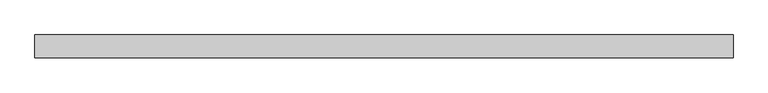
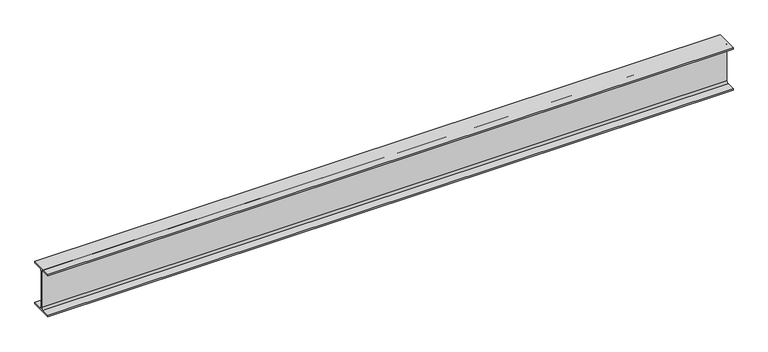
"""IFC4 building model written with IfcOpenShell, lengths in millimetres: beam geometry, 0912_Steel Framing_H-KSD3502 : H_SB_ASB_H-250x125x6x9."""

from ifc_helpers import new_model, si_unit, point, frame, frame_2d, origin, place, context, project, spatial, polyline, circle_curve, trimmed, segment, composite_curve, outline, extrude, source, transform, mapped, element, save


def beam_51e572f2(model_context):
    return source(origin(), model_context, "Body", "SweptSolid", [
        extrude(outline(composite_curve([segment(polyline([(62.5, -116.0), (62.5, -125.0), (-62.5, -125.0), (-62.5, -116.0), (-15.0, -116.0)]), True, "CONTINUOUS"), segment(trimmed(circle_curve(frame_2d((-15.0, -104.0)), 12.0), [point((-15.0, -116.0))], [point((-3.0, -104.0))], True, "CARTESIAN"), True, "CONTINUOUS"), segment(polyline([(-3.0, -104.0), (-3.0, 104.0)]), True, "CONTINUOUS"), segment(trimmed(circle_curve(frame_2d((-15.0, 104.0)), 12.0), [point((-3.0, 104.0))], [point((-15.0, 116.0))], True, "CARTESIAN"), True, "CONTINUOUS"), segment(polyline([(-15.0, 116.0), (-62.5, 116.0), (-62.5, 125.0), (62.5, 125.0), (62.5, 116.0), (15.0, 116.0)]), True, "CONTINUOUS"), segment(trimmed(circle_curve(frame_2d((15.0, 104.0)), 12.0), [point((15.0, 116.0))], [point((3.0, 104.0))], True, "CARTESIAN"), True, "CONTINUOUS"), segment(polyline([(3.0, 104.0), (3.0, -104.0)]), True, "CONTINUOUS"), segment(trimmed(circle_curve(frame_2d((15.0, -104.0)), 12.0), [point((3.0, -104.0))], [point((15.0, -116.0))], True, "CARTESIAN"), True, "CONTINUOUS"), segment(polyline([(15.0, -116.0), (62.5, -116.0)]), True, "CONTINUOUS")], self_intersect=False)), frame((-1904.8, 0.0, 0.0), z_axis=(1.0, 0.0, 0.0), x_axis=(0.0, 1.0, 0.0)), (0.0, 0.0, 1.0), 3809.6),
    ])


if __name__ == "__main__":
    model = new_model("IFC4")
    model_context = context("Model", 3, world=origin())
    ifc_project = project(units=[si_unit("LENGTHUNIT", "METRE", prefix="MILLI")], contexts=[model_context])
    site = spatial("IfcSite", under=ifc_project)
    building = spatial("IfcBuilding", under=site)
    placement = place(None, origin())
    beam_shape = beam_51e572f2(model_context)
    element("IfcBeam", 1, ObjectType="0912_Steel Framing_H-KSD3502 : H_SB_ASB_H-250x125x6x9", at=placement, inside=building, context=model_context, shape_type="MappedRepresentation", body=[
        mapped(beam_shape, transform((0.0, 0.0, 0.0), x_axis=(1.0, 0.0, 0.0), y_axis=(0.0, 1.0, 0.0), z_axis=(0.0, 0.0, 1.0))),
    ])
    save(model, "model.ifc")

# Revit data of these elements
# Type "0912_Steel Framing_H-KSD3502 : H_SB_ASB_H-250x125x6x9"
#   H_WM Code_1 = "S01AA003-00001 | Main Steel Structure Fabrication Work | Shelter/Building | Light Steel - Standard (30KG/M>Weight) | Material: (   )"
#   H_WM Code_2 = "S03AA029-00001 | Main Steel Structure Erection Work | Shelter/Building | Light Steel (30KG/M>Weight) | Material: (   )"
#   H_WM Code_3 = "S01AA010-00001 | Main Steel Structure Fabrication Work | Shelter/Building | Steel Painting/Coating | for Non-Fireproofed Steel Surface, Surface Preparation, Primer, Second & Final Coat | Material: (   )"
#   H_Q'ty Cal Type Tag = "SB-Q2"
#   Width = 12.5 cm
#   Web Thickness = 0.6 cm
#   Web Fillet = 1.2 cm
#   Warping Constant = 42539.8 cm⁶
#   W = 0
#   Torsional Moment of Inertia = 7.8102 cm⁴
#   Section Area = 37.66 cm²
#   Plastic Modulus weak axis = 73.1 cm³
#   Plastic Modulus strong axis = 366.0 cm³
#   Perimeter = 0.97 m²/m
#   Nominal Weight = 29.60 kgf/m
#   Moment of Inertia weak axis = 294.00 cm⁴
#   Moment of Inertia strong axis = 4050.00 cm⁴
#   Height = 25.0 cm
#   Flange Thickness = 0.9 cm
#   Elastic Modulus weak axis = 47.0 cm³
#   Elastic Modulus strong axis = 324.0 cm³
#   Centroid Vertical = 12.5 cm
#   Centroid Horizontal = 6.25 cm
#   Ix = 40500000
#   Length [instance default] = 1.5240 m
#   Zx = 366000
#   b = 0.1250 m
#   h = 0.2500 m
#   r = 0.0120 m
#   s = 0.0060 m
#   t = 0.0090 m
#   A = 0.003766 m²
#   Structural Material [instance default] = Steel, 45-345
#   Assembly Code = ""
# Element 1 (IfcBeam, "0912_Steel Framing_H-KSD3502 : H_SB_ASB_H-250x125x6x9")
#   Structural Material = none
# Materials
#   "Steel, 45-345": class "Metal", colour RGB 189 187 185, transparency 0, Description = "Steel 345 MPa", Cost = 0
